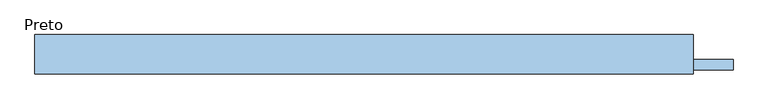
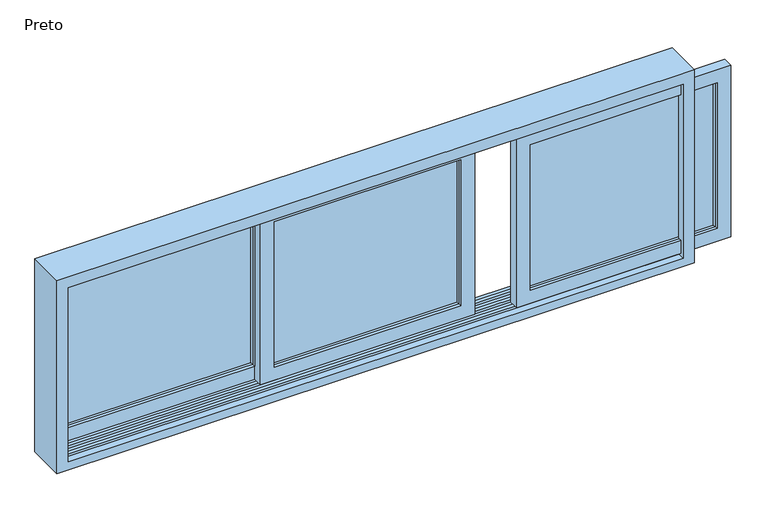
"""IFC4 building model written with IfcOpenShell, lengths in millimetres: window geometry, Blks_Cons Weiku_Janela de Correr 03 Folhas : Preto."""

from ifc_helpers import new_model, si_unit, frame, origin, place, context, project, spatial, polyline, outline, extrude, faceted_brep, source, transform, mapped, element, save


def preto_dc0221ff(model_context):
    return source(origin(), model_context, "Body", "SolidModel", [
        faceted_brep([(-1152.0, 47.0, 898.0), (-1152.0, 42.0, 898.0), (-1152.0, 42.0, 1502.0), (-1152.0, 47.0, 1502.0), (-1147.0, 42.0, 903.0), (-1147.0, 42.0, 1497.0), (-420.0, 42.0, 1502.0), (-420.0, 47.0, 1502.0), (-425.0, 42.0, 1497.0), (-420.0, 42.0, 898.0), (-420.0, 47.0, 898.0), (-425.0, 42.0, 903.0)], [[[0, 1, 2, 3]], [[4, 0, 3, 5]], [[3, 2, 6, 7]], [[5, 3, 7, 8]], [[7, 6, 9, 10]], [[8, 7, 10, 11]], [[1, 9, 6, 2], [5, 8, 11, 4]], [[10, 9, 1, 0]], [[11, 10, 0, 4]]]),
        faceted_brep([(-420.0, 33.0, 898.0), (-420.0, 38.0, 898.0), (-420.0, 38.0, 1502.0), (-420.0, 33.0, 1502.0), (-1152.0, 38.0, 1502.0), (-1152.0, 33.0, 1502.0), (-1152.0, 38.0, 898.0), (-1152.0, 33.0, 898.0), (-425.0, 38.0, 1497.0), (-1147.0, 38.0, 1497.0), (-1147.0, 38.0, 903.0), (-425.0, 38.0, 903.0)], [[[0, 1, 2, 3]], [[3, 2, 4, 5]], [[5, 4, 6, 7]], [[1, 6, 4, 2], [8, 9, 10, 11]], [[7, 6, 1, 0]], [[11, 0, 3, 8]], [[8, 3, 5, 9]], [[9, 5, 7, 10]], [[10, 7, 0, 11]]]),
        extrude(outline(polyline([(-420.0, 38.0), (-1152.0, 38.0), (-1152.0, 42.0), (-420.0, 42.0), (-420.0, 38.0)])), frame((0.0, 0.0, 898.0), z_axis=(0.0, 0.0, 1.0), x_axis=(1.0, 0.0, 0.0)), (0.0, 0.0, 1.0), 604.0),
        extrude(outline(polyline([(844.0, -366.0), (1556.0, -366.0), (1556.0, -1206.0), (844.0, -1206.0), (844.0, -366.0)]), holes=[polyline([(1502.0, -1152.0), (1502.0, -420.0), (898.0, -420.0), (898.0, -1152.0), (1502.0, -1152.0)])]), frame((0.0, 20.0, 0.0), z_axis=(0.0, 1.0, 0.0), x_axis=(0.0, 0.0, 1.0)), (0.0, 0.0, 1.0), 40.0),
        faceted_brep([(-366.0, 7.0, 898.0), (-366.0, 2.0, 898.0), (-366.0, 2.0, 1502.0), (-366.0, 7.0, 1502.0), (-361.0, 2.0, 903.0), (-361.0, 2.0, 1497.0), (366.0, 2.0, 1502.0), (366.0, 7.0, 1502.0), (361.0, 2.0, 1497.0), (366.0, 2.0, 898.0), (366.0, 7.0, 898.0), (361.0, 2.0, 903.0)], [[[0, 1, 2, 3]], [[4, 0, 3, 5]], [[3, 2, 6, 7]], [[5, 3, 7, 8]], [[7, 6, 9, 10]], [[8, 7, 10, 11]], [[1, 9, 6, 2], [5, 8, 11, 4]], [[10, 9, 1, 0]], [[11, 10, 0, 4]]]),
        faceted_brep([(366.0, -7.0, 898.0), (366.0, -2.0, 898.0), (366.0, -2.0, 1502.0), (366.0, -7.0, 1502.0), (-366.0, -2.0, 1502.0), (-366.0, -7.0, 1502.0), (-366.0, -2.0, 898.0), (-366.0, -7.0, 898.0), (361.0, -2.0, 1497.0), (-361.0, -2.0, 1497.0), (-361.0, -2.0, 903.0), (361.0, -2.0, 903.0)], [[[0, 1, 2, 3]], [[3, 2, 4, 5]], [[5, 4, 6, 7]], [[1, 6, 4, 2], [8, 9, 10, 11]], [[7, 6, 1, 0]], [[11, 0, 3, 8]], [[8, 3, 5, 9]], [[9, 5, 7, 10]], [[10, 7, 0, 11]]]),
        extrude(outline(polyline([(366.0, -2.0), (-366.0, -2.0), (-366.0, 2.0), (366.0, 2.0), (366.0, -2.0)])), frame((0.0, 0.0, 898.0), z_axis=(0.0, 0.0, 1.0), x_axis=(1.0, 0.0, 0.0)), (0.0, 0.0, 1.0), 604.0),
        extrude(outline(polyline([(844.0, 420.0), (1556.0, 420.0), (1556.0, -420.0), (844.0, -420.0), (844.0, 420.0)]), holes=[polyline([(1502.0, -366.0), (1502.0, 366.0), (898.0, 366.0), (898.0, -366.0), (1502.0, -366.0)])]), frame((0.0, -20.0, 0.0), z_axis=(0.0, 1.0, 0.0), x_axis=(0.0, 0.0, 1.0)), (0.0, 0.0, 1.0), 40.0),
        faceted_brep([(616.0, -33.0, 898.0), (616.0, -38.0, 898.0), (616.0, -38.0, 1502.0), (616.0, -33.0, 1502.0), (621.0, -38.0, 903.0), (621.0, -38.0, 1497.0), (1348.0, -38.0, 1502.0), (1348.0, -33.0, 1502.0), (1343.0, -38.0, 1497.0), (1348.0, -38.0, 898.0), (1348.0, -33.0, 898.0), (1343.0, -38.0, 903.0)], [[[0, 1, 2, 3]], [[4, 0, 3, 5]], [[3, 2, 6, 7]], [[5, 3, 7, 8]], [[7, 6, 9, 10]], [[8, 7, 10, 11]], [[1, 9, 6, 2], [5, 8, 11, 4]], [[10, 9, 1, 0]], [[11, 10, 0, 4]]]),
        faceted_brep([(1348.0, -47.0, 898.0), (1348.0, -42.0, 898.0), (1348.0, -42.0, 1502.0), (1348.0, -47.0, 1502.0), (616.0, -42.0, 1502.0), (616.0, -47.0, 1502.0), (616.0, -42.0, 898.0), (616.0, -47.0, 898.0), (1343.0, -42.0, 1497.0), (621.0, -42.0, 1497.0), (621.0, -42.0, 903.0), (1343.0, -42.0, 903.0)], [[[0, 1, 2, 3]], [[3, 2, 4, 5]], [[5, 4, 6, 7]], [[1, 6, 4, 2], [8, 9, 10, 11]], [[7, 6, 1, 0]], [[11, 0, 3, 8]], [[8, 3, 5, 9]], [[9, 5, 7, 10]], [[10, 7, 0, 11]]]),
        extrude(outline(polyline([(1348.0, -42.0), (616.0, -42.0), (616.0, -38.0), (1348.0, -38.0), (1348.0, -42.0)])), frame((0.0, 0.0, 898.0), z_axis=(0.0, 0.0, 1.0), x_axis=(1.0, 0.0, 0.0)), (0.0, 0.0, 1.0), 604.0),
        extrude(outline(polyline([(844.0, 1402.0), (1556.0, 1402.0), (1556.0, 562.0), (844.0, 562.0), (844.0, 1402.0)]), holes=[polyline([(1502.0, 616.0), (1502.0, 1348.0), (898.0, 1348.0), (898.0, 616.0), (1502.0, 616.0)])]), frame((0.0, -60.0, 0.0), z_axis=(0.0, 1.0, 0.0), x_axis=(0.0, 0.0, 1.0)), (0.0, 0.0, 1.0), 40.0),
        faceted_brep([(-1206.0, -33.0, 844.0), (-1206.0, -47.0, 844.0), (1206.0, -47.0, 844.0), (1206.0, -33.0, 844.0), (-1206.0, 7.0, 844.0), (-1206.0, -7.0, 844.0), (1206.0, -7.0, 844.0), (1206.0, 7.0, 844.0), (-1206.0, 47.0, 844.0), (-1206.0, 33.0, 844.0), (1206.0, 33.0, 844.0), (1206.0, 47.0, 844.0), (-1206.0, -33.0, 834.0), (-1206.0, -7.0, 834.0), (-1206.0, 7.0, 834.0), (-1206.0, 33.0, 834.0), (-1206.0, 47.0, 834.0), (-1206.0, 75.0, 834.0), (-1206.0, 75.0, 1556.0), (-1206.0, 60.0, 1556.0), (-1206.0, 60.0, 1566.0), (-1206.0, 42.0, 1566.0), (-1206.0, 42.0, 1556.0), (-1206.0, 28.0, 1556.0), (-1206.0, 28.0, 1566.0), (-1206.0, 2.0, 1566.0), (-1206.0, 2.0, 1556.0), (-1206.0, -12.0, 1556.0), (-1206.0, -12.0, 1566.0), (-1206.0, -38.0, 1566.0), (-1206.0, -38.0, 1556.0), (-1206.0, -52.0, 1556.0), (-1206.0, -52.0, 1566.0), (-1206.0, -60.0, 1566.0), (-1206.0, -60.0, 1556.0), (-1206.0, -75.0, 1556.0), (-1206.0, -75.0, 834.0), (-1206.0, -47.0, 834.0), (1206.0, -47.0, 834.0), (1206.0, -12.0, 1556.0), (1206.0, 2.0, 1556.0), (1206.0, 2.0, 1566.0), (1206.0, 28.0, 1566.0), (1206.0, 28.0, 1556.0), (1206.0, 42.0, 1556.0), (1206.0, 42.0, 1566.0), (1206.0, 60.0, 1566.0), (1206.0, 60.0, 1556.0), (1206.0, 75.0, 1556.0), (1206.0, 75.0, 834.0), (1206.0, 47.0, 834.0), (1206.0, 33.0, 834.0), (1206.0, 7.0, 834.0), (1206.0, -7.0, 834.0), (1206.0, -33.0, 834.0), (1206.0, -75.0, 834.0), (1206.0, -75.0, 1556.0), (1206.0, -60.0, 1556.0), (1206.0, -60.0, 1566.0), (1206.0, -52.0, 1566.0), (1206.0, -52.0, 1556.0), (1206.0, -38.0, 1556.0), (1206.0, -38.0, 1566.0), (1206.0, -12.0, 1566.0), (1250.0, -75.0, 800.0), (1250.0, 75.0, 800.0), (1250.0, 75.0, 1600.0), (1250.0, -75.0, 1600.0), (-1250.0, -75.0, 800.0), (-1250.0, 75.0, 800.0), (-1250.0, -75.0, 1600.0), (-1250.0, 75.0, 1600.0)], [[[0, 1, 2, 3]], [[4, 5, 6, 7]], [[8, 9, 10, 11]], [[1, 0, 12, 13, 5, 4, 14, 15, 9, 8, 16, 17, 18, 19, 20, 21, 22, 23, 24, 25, 26, 27, 28, 29, 30, 31, 32, 33, 34, 35, 36, 37]], [[38, 2, 1, 37]], [[39, 40, 41, 42, 43, 44, 45, 46, 47, 48, 49, 50, 11, 10, 51, 52, 7, 6, 53, 54, 3, 2, 38, 55, 56, 57, 58, 59, 60, 61, 62, 63]], [[3, 54, 12, 0]], [[53, 6, 5, 13]], [[7, 52, 14, 4]], [[51, 10, 9, 15]], [[11, 50, 16, 8]], [[64, 65, 66, 67]], [[65, 64, 68, 69]], [[68, 64, 67, 70], [36, 35, 56, 55]], [[69, 68, 70, 71]], [[65, 69, 71, 66], [49, 48, 18, 17]], [[54, 53, 13, 12]], [[52, 51, 15, 14]], [[50, 49, 17, 16]], [[55, 38, 37, 36]], [[23, 22, 44, 43]], [[27, 26, 40, 39]], [[31, 30, 61, 60]], [[18, 48, 47, 19]], [[56, 35, 34, 57]], [[71, 70, 67, 66]], [[43, 42, 24, 23]], [[42, 41, 25, 24]], [[41, 40, 26, 25]], [[39, 63, 28, 27]], [[63, 62, 29, 28]], [[62, 61, 30, 29]], [[60, 59, 32, 31]], [[59, 58, 33, 32]], [[33, 58, 57, 34]], [[46, 20, 19, 47]], [[46, 45, 21, 20]], [[45, 44, 22, 21]]]),
    ])


if __name__ == "__main__":
    model = new_model("IFC4")
    model_context = context("Model", 3, world=origin())
    ifc_project = project(units=[si_unit("LENGTHUNIT", "METRE", prefix="MILLI")], contexts=[model_context])
    site = spatial("IfcSite", under=ifc_project)
    building = spatial("IfcBuilding", under=site)
    placement = place(None, origin())
    preto_shape = preto_dc0221ff(model_context)
    element("IfcWindow", 1, ObjectType="Blks_Cons Weiku_Janela de Correr 03 Folhas : Preto", at=placement, inside=building, context=model_context, shape_type="MappedRepresentation", body=[
        mapped(preto_shape, transform((0.0, 0.0, 0.0), x_axis=(1.0, 0.0, 0.0), y_axis=(0.0, 1.0, 0.0), z_axis=(0.0, 0.0, 1.0))),
    ])
    save(model, "model.ifc")

# Revit data of these elements
# Type "Blks_Cons Weiku_Janela de Correr 03 Folhas : Preto"
#   Type Mark = "J23"
#   Type Comments = "Janela de Correr 03 Folhas"
#   Manufacturer = "Weiku"
#   Created By / Criado Por / Creado por = "Blocks"
#   Author URL = "https://BlocksRvt.com/"
#   Author Contact = "info@blocksrvt.com"
#   Assembly Code = "Cons"
#   b [instance default] = 912 mm
#   a [instance default] = 1036 mm
#   Width [instance default] = 3000 mm
#   Rough Width [instance default] = 3088 mm
#   Rough Height [instance default] = 1000 mm
#   Height [instance default] = 912 mm
#   Espessura Folha [instance default] = 40 mm
#   Abertura Folha Interna [instance default] = 75 mm
#   Abertura Folha Externa [instance default] = 1964 mm
#   Abertura Folha Central [instance default] = 982 mm
#   Vidro = .vidro_growarq
#   Vedação = Blks - Rubber - Black
#   Janela = Blks - Plastic - Black - Glazed
#   Wall Closure = (empty or 0)
# Element 1 (IfcWindow, "Blks_Cons Weiku_Janela de Correr 03 Folhas : Preto")
#   b = 712 mm
#   a = 840 mm
#   Width = 2412 mm
#   Rough Width = 2500 mm
#   Rough Height = 800 mm
#   Height = 712 mm
#   Abertura Folha Interna = 0 mm
#   Abertura Folha Externa = 400 mm
#   Abertura Folha Central = 600 mm
#   Materials on its faces: "Blks - Plastic - Black - Glazed", "Blks - Rubber - Black", ".vidro_growarq"
# Materials
#   ".vidro_growarq": class "Vidro", colour RGB 200 215 215, transparency 0.6, Description = "Vidroverde", Cost = 0
#   "Blks - Rubber - Black": class "Paint/Coating", colour RGB 38 38 38, transparency 0, Cost = 0
#   "Blks - Plastic - Black - Glazed": class "Plastic", colour RGB 25 25 25, transparency 0, Cost = 0
